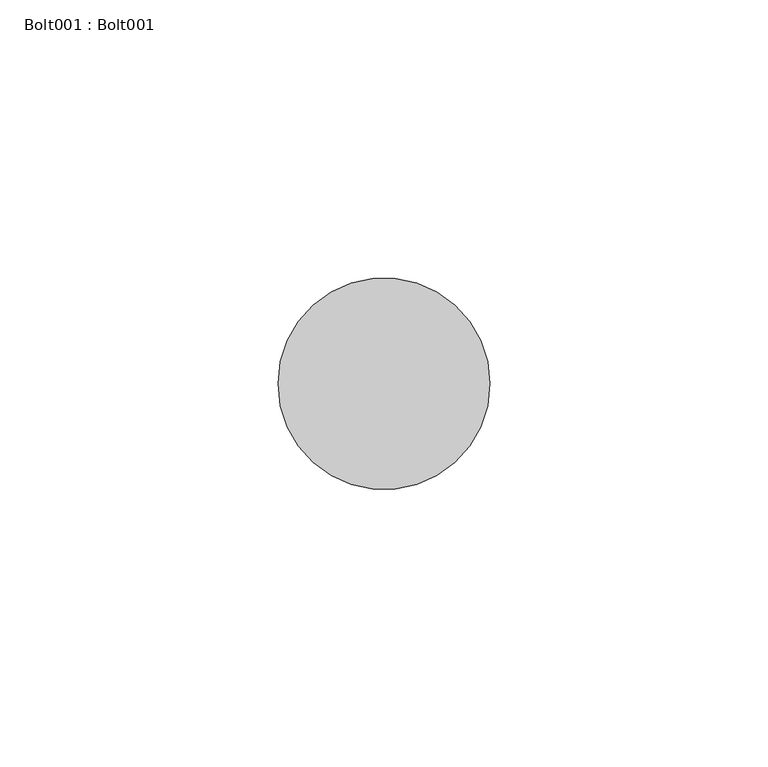
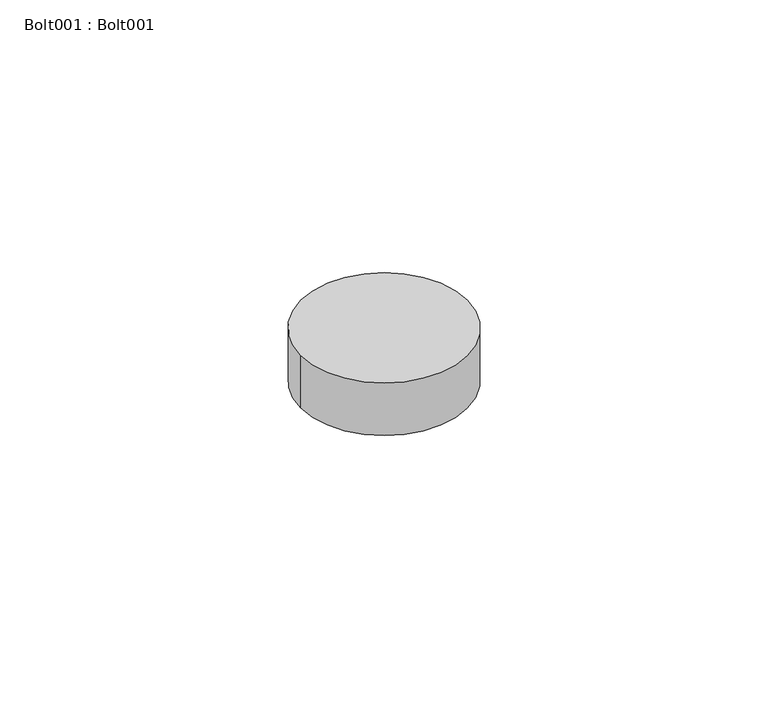
"""IFC4 building model written with IfcOpenShell, lengths in millimetres: proxy geometry, Bolt001 : Bolt001."""

from ifc_helpers import new_model, si_unit, point, frame, frame_2d, origin, place, context, project, spatial, circle_curve, trimmed, segment, composite_curve, outline, extrude, source, transform, mapped, element, save


def bolt001_bolt001_70c8ac4d(model_context):
    return source(origin(), model_context, "Body", "SweptSolid", [
        extrude(outline(composite_curve([segment(trimmed(circle_curve(frame_2d((7251.9702148, -1781.8449707)), 19.05), [point((7232.9202148, -1781.8449707))], [point((7271.0202148, -1781.8449707))], False, "CARTESIAN"), True, "CONTINUOUS"), segment(trimmed(circle_curve(frame_2d((7251.9702148, -1781.8449707)), 19.05), [point((7271.0202148, -1781.8449707))], [point((7232.9202148, -1781.8449707))], False, "CARTESIAN"), True, "CONTINUOUS")], self_intersect=False)), frame((0.0, 0.0, 40112.696), z_axis=(0.0, 0.0, 1.0), x_axis=(1.0, 0.0, 0.0)), (0.0, 0.0, 1.0), 12.7),
    ])


if __name__ == "__main__":
    model = new_model("IFC4")
    model_context = context("Model", 3, world=origin())
    ifc_project = project(units=[si_unit("LENGTHUNIT", "METRE", prefix="MILLI")], contexts=[model_context])
    site = spatial("IfcSite", under=ifc_project)
    building = spatial("IfcBuilding", under=site)
    placement = place(None, origin())
    bolt001_bolt001_shape = bolt001_bolt001_70c8ac4d(model_context)
    element("IfcBuildingElementProxy", 1, Name="Bolt001 : Bolt001", ObjectType="Bolt001 : Bolt001", at=placement, inside=building, context=model_context, shape_type="MappedRepresentation", body=[
        mapped(bolt001_bolt001_shape, transform((0.0, 0.0, 0.0), x_axis=(1.0, 0.0, 0.0), y_axis=(0.0, 1.0, 0.0), z_axis=(0.0, 0.0, 1.0))),
    ])
    save(model, "model.ifc")

# Revit data of these elements
# Type "Bolt001 : Bolt001"
#   NameOverride = "Bolt001"
# Element 1 (IfcBuildingElementProxy, "Bolt001 : Bolt001")
#   Materials on its faces: "BOLTS CONCEALED BY FLOOR FINISH"
# Materials
#   "BOLTS CONCEALED BY FLOOR FINISH": class "Unassigned", colour RGB 128 128 128, transparency 0
